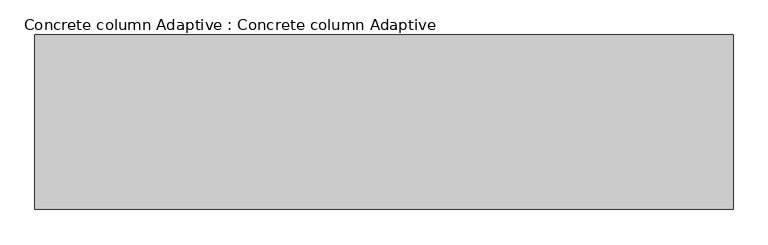
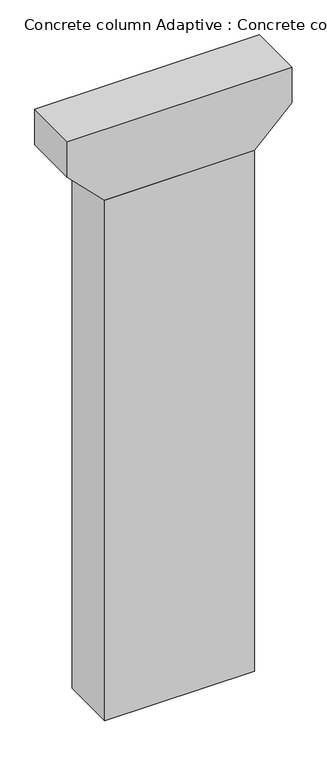
"""IFC4 building model written with IfcOpenShell, lengths in millimetres: proxy geometry, Concrete column Adaptive : Concrete column Adaptive."""

from ifc_helpers import new_model, si_unit, frame, origin, origin_with_axes, place, context, project, spatial, polyline, outline, extrude, source, transform, mapped, element, save


def concrete_column_adaptive_concrete_column_adaptive_c5f28f15(model_context):
    return source(origin(), model_context, "Body", "SweptSolid", [
        extrude(outline(polyline([(33382.0, 6000.0), (33382.0, -6000.0), (31382.0, -6000.0), (29382.0, -4000.0), (29382.0, 4000.0), (31382.0, 6000.0), (33382.0, 6000.0)])), frame((0.0, -1500.0, 0.0), z_axis=(0.0, 1.0, 0.0), x_axis=(0.0, 0.0, 1.0)), (0.0, 0.0, 1.0), 3000.0),
        extrude(outline(polyline([(-4000.0, -1500.0), (-4000.0, 1500.0), (4000.0, 1500.0), (4000.0, -1500.0), (-4000.0, -1500.0)])), origin_with_axes(), (0.0, 0.0, 1.0), 29382.0),
    ])


if __name__ == "__main__":
    model = new_model("IFC4")
    model_context = context("Model", 3, world=origin())
    ifc_project = project(units=[si_unit("LENGTHUNIT", "METRE", prefix="MILLI")], contexts=[model_context])
    site = spatial("IfcSite", under=ifc_project)
    building = spatial("IfcBuilding", under=site)
    placement = place(None, origin())
    concrete_column_adaptive_concrete_column_adaptive_shape = concrete_column_adaptive_concrete_column_adaptive_c5f28f15(model_context)
    element("IfcBuildingElementProxy", 1, Name="Concrete column Adaptive : Concrete column Adaptive", ObjectType="Concrete column Adaptive : Concrete column Adaptive", at=placement, inside=building, context=model_context, shape_type="MappedRepresentation", body=[
        mapped(concrete_column_adaptive_concrete_column_adaptive_shape, transform((0.0, 0.0, 0.0), x_axis=(1.0, 0.0, 0.0), y_axis=(0.0, 1.0, 0.0), z_axis=(0.0, 0.0, 1.0))),
    ])
    save(model, "model.ifc")

# Revit data of these elements
# Type "Concrete column Adaptive : Concrete column Adaptive"
#   Height [instance default] = 30000 mm
#   Default Elevation = 0
# Element 1 (IfcBuildingElementProxy, "Concrete column Adaptive : Concrete column Adaptive")
#   Height = 29382 mm
